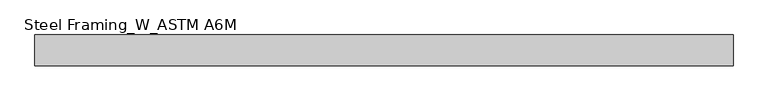
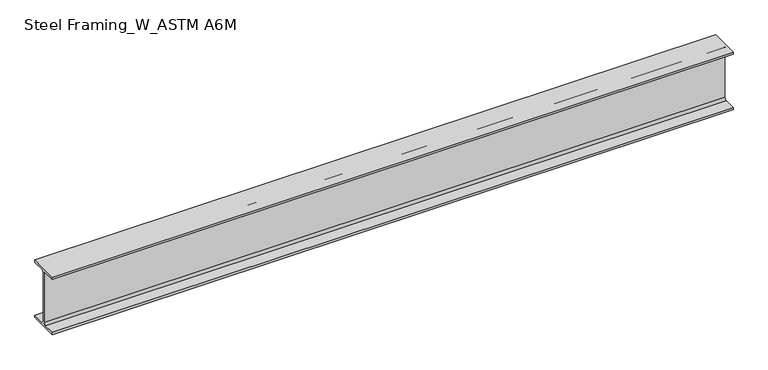
"""IFC4 building model written with IfcOpenShell, lengths in millimetres: beam geometry, Steel Framing_W_ASTM A6M : H_SB_AR_S02_W200x22.5_B7."""

from ifc_helpers import new_model, si_unit, point, frame, frame_2d, origin, place, context, project, spatial, polyline, circle_curve, trimmed, segment, composite_curve, outline, extrude, source, transform, mapped, element, save


def steel_framing_w_astm_a6m_683fa1ff(model_context):
    return source(origin(), model_context, "Body", "SweptSolid", [
        extrude(outline(composite_curve([segment(polyline([(51.0, -95.0), (51.0, -103.0), (-51.0, -103.0), (-51.0, -95.0), (-10.71, -95.0)]), True, "CONTINUOUS"), segment(trimmed(circle_curve(frame_2d((-10.71, -87.4)), 7.6), [point((-10.71, -95.0))], [point((-3.11, -87.4))], True, "CARTESIAN"), True, "CONTINUOUS"), segment(polyline([(-3.11, -87.4), (-3.11, 87.4)]), True, "CONTINUOUS"), segment(trimmed(circle_curve(frame_2d((-10.71, 87.4)), 7.6), [point((-3.11, 87.4))], [point((-10.71, 95.0))], True, "CARTESIAN"), True, "CONTINUOUS"), segment(polyline([(-10.71, 95.0), (-51.0, 95.0), (-51.0, 103.0), (51.0, 103.0), (51.0, 95.0), (10.71, 95.0)]), True, "CONTINUOUS"), segment(trimmed(circle_curve(frame_2d((10.71, 87.4)), 7.6), [point((10.71, 95.0))], [point((3.11, 87.4))], True, "CARTESIAN"), True, "CONTINUOUS"), segment(polyline([(3.11, 87.4), (3.11, -87.4)]), True, "CONTINUOUS"), segment(trimmed(circle_curve(frame_2d((10.71, -87.4)), 7.6), [point((3.11, -87.4))], [point((10.71, -95.0))], True, "CARTESIAN"), True, "CONTINUOUS"), segment(polyline([(10.71, -95.0), (51.0, -95.0)]), True, "CONTINUOUS")], self_intersect=False)), frame((-1151.8, 0.0, 0.0), z_axis=(1.0, 0.0, 0.0), x_axis=(0.0, 1.0, 0.0)), (0.0, 0.0, 1.0), 2303.6),
    ])


if __name__ == "__main__":
    model = new_model("IFC4")
    model_context = context("Model", 3, world=origin())
    ifc_project = project(units=[si_unit("LENGTHUNIT", "METRE", prefix="MILLI")], contexts=[model_context])
    site = spatial("IfcSite", under=ifc_project)
    building = spatial("IfcBuilding", under=site)
    placement = place(None, origin())
    steel_framing_w_astm_a6m_shape = steel_framing_w_astm_a6m_683fa1ff(model_context)
    element("IfcBeam", 1, ObjectType="Steel Framing_W_ASTM A6M : H_SB_AR_S02_W200x22.5_B7", at=placement, inside=building, context=model_context, shape_type="MappedRepresentation", body=[
        mapped(steel_framing_w_astm_a6m_shape, transform((0.0, 0.0, 0.0), x_axis=(1.0, 0.0, 0.0), y_axis=(0.0, 1.0, 0.0), z_axis=(0.0, 0.0, 1.0))),
    ])
    save(model, "model.ifc")

# Revit data of these elements
# Type "Steel Framing_W_ASTM A6M : H_SB_AR_S02_W200x22.5_B7"
#   Type Mark = "B7"
#   Section Name Key = "W8x15"
#   Width = 10.2 cm
#   Web Thickness = 0.622 cm
#   Web Fillet = 0.76 cm
#   Warping Constant = 13900.0 cm⁶
#   Torsional Moment of Inertia = 5.70 cm⁴
#   Section Area = 28.6 cm²
#   Plastic Modulus weak axis = 43.8 cm³
#   Plastic Modulus strong axis = 223.0 cm³
#   Perimeter = 0.795 m²/m
#   Nominal Weight = 22.50 kgf/m
#   Moment of Inertia weak axis = 142.00 cm⁴
#   Moment of Inertia strong axis = 2000.00 cm⁴
#   Height = 20.6 cm
#   Flange Thickness = 0.8 cm
#   Elastic Modulus weak axis = 27.9 cm³
#   Elastic Modulus strong axis = 193.0 cm³
#   Centroid Vertical = 10.3 cm
#   Centroid Horizontal = 5.1 cm
#   Length [instance default] = 1500 mm
#   Structural Material [instance default] = Steel, 45-345
#   Bolt Spacing = 0
#   Assembly Code = ""
# Element 1 (IfcBeam, "Steel Framing_W_ASTM A6M : H_SB_AR_S02_W200x22.5_B7")
#   Materials on its faces: "Steel, 45-345"
# Materials
#   "Steel, 45-345": class "Metal", colour RGB 189 187 185, transparency 0, Description = "Steel 345 MPa", Cost = 0
